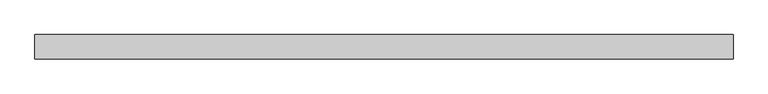
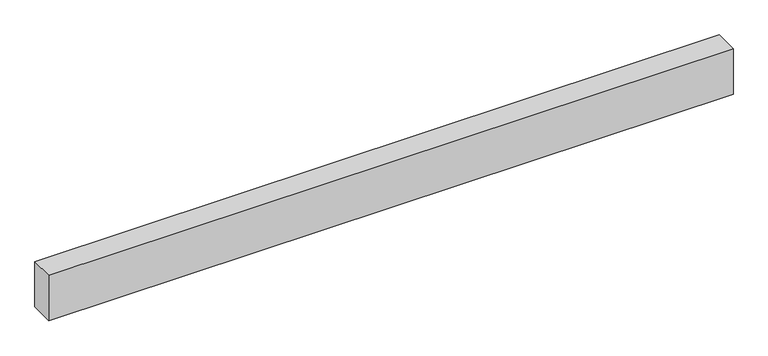
"""IFC4 building model written with IfcOpenShell, lengths in millimetres: beam geometry, Madeira de lei : Berço 6x12cm."""

import ifcopenshell
import ifcopenshell.guid

model = None  # the IFC model being written
_history = None  # IfcOwnerHistory: only IFC2X3 demands one
_inside = {}  # id of a spatial element -> (the spatial element, [elements in it])
_under = {}  # id of a project, library or spatial element -> (it, [spatial elements below it])
_declared = {}  # id of a project -> (the project, [libraries it declares])
_typed = {}  # id of a type object -> (the type object, [elements of that type])
_made_of = {}  # id of a material, layer set ... -> (it, [elements and type objects made of it])


def new_model(schema):
    """Start an empty IFC model of exactly this schema.

    Asked for "IFC4X3", IfcOpenShell would pick the latest addendum, in which some entities
    have other attributes; the version numbers below select the first issue.
    IFC2X3 requires an IfcOwnerHistory on every rooted entity: one is made here for all.
    """
    global model, _history
    if schema == "IFC4X3":
        model = ifcopenshell.file(schema_version=(4, 3, 0, 0))
    else:
        model = ifcopenshell.file(schema=schema)
    _inside.clear()
    _under.clear()
    _declared.clear()
    _typed.clear()
    _made_of.clear()
    _history = None
    if model.schema == "IFC2X3":
        org = make("IfcOrganization", Name="unknown")
        user = make(
            "IfcPersonAndOrganization",
            ThePerson=make("IfcPerson", FamilyName="unknown"),
            TheOrganization=org,
        )
        app = make(
            "IfcApplication",
            ApplicationDeveloper=org,
            Version="unknown",
            ApplicationFullName="unknown",
            ApplicationIdentifier="unknown",
        )
        _history = make(
            "IfcOwnerHistory",
            OwningUser=user,
            OwningApplication=app,
            ChangeAction="ADDED",
            CreationDate=0,
        )
    return model


def make(cls, **values):
    """One entity of the class cls with the attributes given. An attribute that is None is left unset."""
    return model.create_entity(
        cls, **{name: value for name, value in values.items() if value is not None}
    )


def rooted(cls, **values):
    """An entity with a GlobalId (a new one), such as an element, a storey or a relation."""
    return make(cls, GlobalId=ifcopenshell.guid.new(), OwnerHistory=_history, **values)


def si_unit(unit_type, name, prefix=None):
    """IfcSIUnit, for example si_unit("LENGTHUNIT", "METRE", prefix="MILLI")."""
    return make("IfcSIUnit", UnitType=unit_type, Prefix=prefix, Name=name)


def assignment(units):
    """IfcUnitAssignment: the units of a project."""
    return None if units is None else make("IfcUnitAssignment", Units=units)


def point(xyz):
    """IfcCartesianPoint."""
    return None if xyz is None else make("IfcCartesianPoint", Coordinates=xyz)


def direction(xyz):
    """IfcDirection."""
    return None if xyz is None else make("IfcDirection", DirectionRatios=xyz)


def frame(location, z_axis=None, x_axis=None):
    """IfcAxis2Placement3D, a coordinate frame: its origin and axes. An axis left out is left unset."""
    return make(
        "IfcAxis2Placement3D",
        Location=point(location),
        Axis=direction(z_axis),
        RefDirection=direction(x_axis),
    )


def origin():
    """The frame at (0, 0, 0) with its axes left unset."""
    return frame((0.0, 0.0, 0.0))


def place(relative_to, where):
    """IfcLocalPlacement: puts the frame where relative to a parent placement (None: the world)."""
    return make(
        "IfcLocalPlacement", PlacementRelTo=relative_to, RelativePlacement=where
    )


def context(
    kind, dimensions, precision=None, world=None, true_north=None, identifier=None
):
    """IfcGeometricRepresentationContext, for example the 3D "Model" context."""
    return make(
        "IfcGeometricRepresentationContext",
        ContextIdentifier=identifier,
        ContextType=kind,
        CoordinateSpaceDimension=dimensions,
        Precision=precision,
        WorldCoordinateSystem=world,
        TrueNorth=true_north,
    )


def project(units=None, contexts=None):
    """IfcProject with its units and contexts."""
    return rooted(
        "IfcProject",
        Name="project",
        RepresentationContexts=contexts,
        UnitsInContext=assignment(units),
    )


def spatial(cls, under=None, at=None, **own):
    """A site, building, storey or space (cls), placed at a placement, below another one or the project."""
    s = rooted(cls, ObjectPlacement=at, **own)
    if under is not None:
        _under.setdefault(under.id(), (under, []))[1].append(s)
    return s


def polyline(points):
    """IfcPolyline through the points."""
    return make("IfcPolyline", Points=[point(p) for p in points])


def outline(outer, holes=None, kind="AREA"):
    """IfcArbitraryClosedProfileDef: a profile drawn as a closed curve; with holes, ...WithVoids."""
    if holes is None:
        return make("IfcArbitraryClosedProfileDef", ProfileType=kind, OuterCurve=outer)
    return make(
        "IfcArbitraryProfileDefWithVoids",
        ProfileType=kind,
        OuterCurve=outer,
        InnerCurves=holes,
    )


def extrude(swept, where, along, depth):
    """IfcExtrudedAreaSolid: the profile swept, set in the frame where, extruded along a direction by depth."""
    return make(
        "IfcExtrudedAreaSolid",
        SweptArea=swept,
        Position=where,
        ExtrudedDirection=direction(along),
        Depth=depth,
    )


def shape(context_of_items, identifier, shape_type, items):
    """IfcShapeRepresentation: the items that make up one representation, for example the "Body"."""
    return make(
        "IfcShapeRepresentation",
        ContextOfItems=context_of_items,
        RepresentationIdentifier=identifier,
        RepresentationType=shape_type,
        Items=items,
    )


def source(mapping_origin, context_of_items, identifier, shape_type, items):
    """IfcRepresentationMap: a shape defined once, which mapped items show again and again."""
    return make(
        "IfcRepresentationMap",
        MappingOrigin=mapping_origin,
        MappedRepresentation=shape(context_of_items, identifier, shape_type, items),
    )


def transform(
    local_origin,
    x_axis=None,
    y_axis=None,
    z_axis=None,
    scale=None,
    scale2=None,
    scale3=None,
    uniform=True,
):
    """IfcCartesianTransformationOperator3D, or its non-uniform kind. x_axis, y_axis, z_axis: its Axis1, 2, 3."""
    if uniform:
        return make(
            "IfcCartesianTransformationOperator3D",
            Axis1=direction(x_axis),
            Axis2=direction(y_axis),
            LocalOrigin=point(local_origin),
            Scale=scale,
            Axis3=direction(z_axis),
        )
    return make(
        "IfcCartesianTransformationOperator3DnonUniform",
        Axis1=direction(x_axis),
        Axis2=direction(y_axis),
        LocalOrigin=point(local_origin),
        Scale=scale,
        Axis3=direction(z_axis),
        Scale2=scale2,
        Scale3=scale3,
    )


def mapped(mapping_source, mapping_target):
    """IfcMappedItem: shows the shape of a source again, moved by a transform."""
    return make(
        "IfcMappedItem", MappingSource=mapping_source, MappingTarget=mapping_target
    )


def made_of(thing, what):
    """Note that an element or type object is made of a material, layer set ...; save() writes the relation."""
    if what is not None:
        _made_of.setdefault(what.id(), (what, []))[1].append(thing)
    return thing


def element(
    cls,
    number,
    at=None,
    inside=None,
    cuts=None,
    type_object=None,
    material=None,
    context=None,
    identifier="Body",
    shape_type=None,
    held_by="IfcProductDefinitionShape",
    body=None,
    shapes=None,
    **own,
):
    """One element of the class cls, such as IfcWall. Its Tag is "e" and its number.

    at: its placement. inside: the storey or other place that contains it. cuts: it is an
    opening in that element (IfcRelVoidsElement). A single representation is given by context,
    identifier, shape_type and body (its items); several are given by shapes. held_by: the class
    of the entity that holds the representations. save() writes the other relations.
    """
    e = rooted(cls, Tag="e%d" % number, ObjectPlacement=at, **own)
    if body is not None:
        shapes = [shape(context, identifier, shape_type, body)]
    if shapes is not None:
        e.Representation = make(held_by, Representations=shapes)
    if inside is not None:
        _inside.setdefault(inside.id(), (inside, []))[1].append(e)
    if cuts is not None:
        rooted(
            "IfcRelVoidsElement", RelatingBuildingElement=cuts, RelatedOpeningElement=e
        )
    if type_object is not None:
        _typed.setdefault(type_object.id(), (type_object, []))[1].append(e)
    return made_of(e, material)


def aggregate(whole, parts):
    """IfcRelAggregates: a whole, such as a stair, and the parts it consists of."""
    return rooted("IfcRelAggregates", RelatingObject=whole, RelatedObjects=parts)


def save(model, path):
    """Write the relations noted so far, then the file.

    IfcRelAggregates (storeys below a building ...), IfcRelContainedInSpatialStructure (elements
    in a storey), IfcRelDefinesByType, IfcRelAssociatesMaterial and IfcRelDeclares: one each for
    every whole, place, type object, material and project.
    """
    for whole, parts in _under.values():
        aggregate(whole, parts)
    for where, things in _inside.values():
        rooted(
            "IfcRelContainedInSpatialStructure",
            RelatedElements=things,
            RelatingStructure=where,
        )
    for kind, things in _typed.values():
        rooted("IfcRelDefinesByType", RelatedObjects=things, RelatingType=kind)
    for what, things in _made_of.values():
        rooted("IfcRelAssociatesMaterial", RelatedObjects=things, RelatingMaterial=what)
    for by, libraries in _declared.values():
        rooted("IfcRelDeclares", RelatingContext=by, RelatedDefinitions=libraries)
    model.write(path)


def beam_739eac5c(model_context):
    return source(origin(), model_context, "Body", "SweptSolid", [
        extrude(outline(polyline([(854.9999994, 30.0), (854.9999994, -30.0), (-855.0, -30.0), (-855.0, 30.0), (854.9999994, 30.0)])), frame((0.0, 0.0, -60.0), z_axis=(0.0, 0.0, 1.0), x_axis=(1.0, 0.0, 0.0)), (0.0, 0.0, 1.0), 120.0),
    ])


if __name__ == "__main__":
    model = new_model("IFC4")
    model_context = context("Model", 3, world=origin())
    ifc_project = project(units=[si_unit("LENGTHUNIT", "METRE", prefix="MILLI")], contexts=[model_context])
    site = spatial("IfcSite", under=ifc_project)
    building = spatial("IfcBuilding", under=site)
    placement = place(None, origin())
    beam_shape = beam_739eac5c(model_context)
    element("IfcBeam", 1, ObjectType="Madeira de lei : Berço 6x12cm", at=placement, inside=building, context=model_context, shape_type="MappedRepresentation", body=[
        mapped(beam_shape, transform((0.0, 0.0, 0.0), x_axis=(1.0, 0.0, 0.0), y_axis=(0.0, 1.0, 0.0), z_axis=(0.0, 0.0, 1.0))),
    ])
    save(model, "model.ifc")

# Revit data of these elements
# Type "Madeira de lei : Berço 6x12cm"
#   A = 0.02 m²
#   Length [instance default] = 1.524 m
#   b = 0.06 m
#   d = 0.12 m
#   Structural Material [instance default] = none
#   Assembly Code = ""
# Element 1 (IfcBeam, "Madeira de lei : Berço 6x12cm")
#   Structural Material = .MADEIRAMENTO
#   Materials on its faces: ".MADEIRAMENTO"
# Materials
#   ".MADEIRAMENTO": class ".CC_MADEIRAS", colour RGB 212 179 113, transparency 0, Cost = 0
